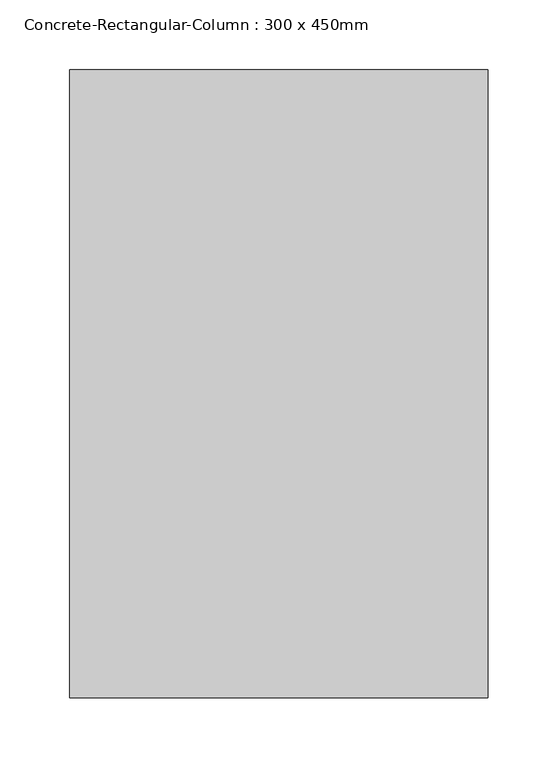
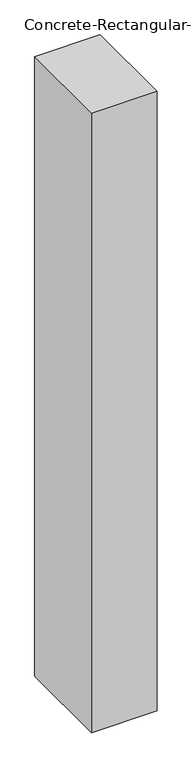
"""IFC4 building model written with IfcOpenShell, lengths in millimetres: column geometry, Concrete-Rectangular-Column : 300 x 450mm."""

from ifc_helpers import new_model, si_unit, origin, origin_with_axes, place, context, project, spatial, polyline, outline, extrude, source, transform, mapped, element, save


def concrete_rectangular_column_300_x_450mm_5cd98a27(model_context):
    return source(origin(), model_context, "Body", "SweptSolid", [
        extrude(outline(polyline([(150.0, 225.0), (150.0, -225.0), (-150.0, -225.0), (-150.0, 225.0), (150.0, 225.0)])), origin_with_axes(), (0.0, 0.0, 1.0), 3000.0),
    ])


if __name__ == "__main__":
    model = new_model("IFC4")
    model_context = context("Model", 3, world=origin())
    ifc_project = project(units=[si_unit("LENGTHUNIT", "METRE", prefix="MILLI")], contexts=[model_context])
    site = spatial("IfcSite", under=ifc_project)
    building = spatial("IfcBuilding", under=site)
    placement = place(None, origin())
    concrete_rectangular_column_300_x_450mm_shape = concrete_rectangular_column_300_x_450mm_5cd98a27(model_context)
    element("IfcColumn", 1, ObjectType="Concrete-Rectangular-Column : 300 x 450mm", at=placement, inside=building, context=model_context, shape_type="MappedRepresentation", body=[
        mapped(concrete_rectangular_column_300_x_450mm_shape, transform((0.0, 0.0, 0.0), x_axis=(1.0, 0.0, 0.0), y_axis=(0.0, 1.0, 0.0), z_axis=(0.0, 0.0, 1.0))),
    ])
    save(model, "model.ifc")

# Revit data of these elements
# Type "Concrete-Rectangular-Column : 300 x 450mm"
#   b = 300 mm
#   h = 450 mm
#   Structural Material [instance default] = Concrete, Cast-in-Place gray
# Element 1 (IfcColumn, "Concrete-Rectangular-Column : 300 x 450mm")
#   Materials on its faces: "Concrete, Cast-in-Place gray"
# Materials
#   "Concrete, Cast-in-Place gray": class "Concrete", colour RGB 192 192 192, transparency 0, Description = "Cast-in-place concrete", Cost = 0
